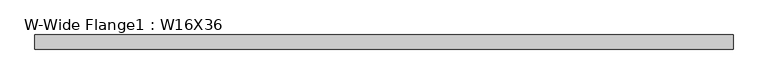
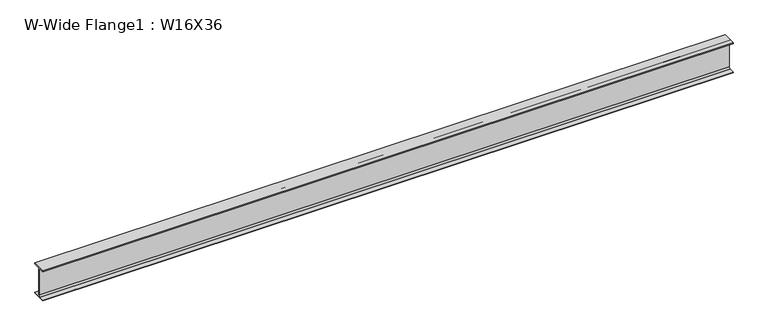
"""IFC4 building model written with IfcOpenShell, lengths in millimetres: beam geometry, W-Wide Flange1 : W16X36."""

from ifc_helpers import new_model, si_unit, point, frame, frame_2d, origin, place, context, project, spatial, polyline, circle_curve, trimmed, segment, composite_curve, outline, extrude, source, transform, mapped, element, save


def w_wide_flange1_w16x36_dd20d998(model_context):
    return source(origin(), model_context, "Body", "SweptSolid", [
        extrude(outline(composite_curve([segment(polyline([(88.773, -191.008), (88.773, -201.93), (-88.773, -201.93), (-88.773, -191.008), (-21.3995, -191.008)]), True, "CONTINUOUS"), segment(trimmed(circle_curve(frame_2d((-21.3995, -173.355)), 17.653), [point((-21.3995, -191.008))], [point((-3.7465, -173.355))], True, "CARTESIAN"), True, "CONTINUOUS"), segment(polyline([(-3.7465, -173.355), (-3.7465, 173.355)]), True, "CONTINUOUS"), segment(trimmed(circle_curve(frame_2d((-21.3995, 173.355)), 17.653), [point((-3.7465, 173.355))], [point((-21.3995, 191.008))], True, "CARTESIAN"), True, "CONTINUOUS"), segment(polyline([(-21.3995, 191.008), (-88.773, 191.008), (-88.773, 201.93), (88.773, 201.93), (88.773, 191.008), (21.3995, 191.008)]), True, "CONTINUOUS"), segment(trimmed(circle_curve(frame_2d((21.3995, 173.355)), 17.653), [point((21.3995, 191.008))], [point((3.7465, 173.355))], True, "CARTESIAN"), True, "CONTINUOUS"), segment(polyline([(3.7465, 173.355), (3.7465, -173.355)]), True, "CONTINUOUS"), segment(trimmed(circle_curve(frame_2d((21.3995, -173.355)), 17.653), [point((3.7465, -173.355))], [point((21.3995, -191.008))], True, "CARTESIAN"), True, "CONTINUOUS"), segment(polyline([(21.3995, -191.008), (88.773, -191.008)]), True, "CONTINUOUS")], self_intersect=False)), frame((-4399.7267802, 0.0, 0.0), z_axis=(1.0, 0.0, 0.0), x_axis=(0.0, 1.0, 0.0)), (0.0, 0.0, 1.0), 8787.9151819),
    ])


if __name__ == "__main__":
    model = new_model("IFC4")
    model_context = context("Model", 3, world=origin())
    ifc_project = project(units=[si_unit("LENGTHUNIT", "METRE", prefix="MILLI")], contexts=[model_context])
    site = spatial("IfcSite", under=ifc_project)
    building = spatial("IfcBuilding", under=site)
    placement = place(None, origin())
    w_wide_flange1_w16x36_shape = w_wide_flange1_w16x36_dd20d998(model_context)
    element("IfcBeam", 1, ObjectType="W-Wide Flange1 : W16X36", at=placement, inside=building, context=model_context, shape_type="MappedRepresentation", body=[
        mapped(w_wide_flange1_w16x36_shape, transform((0.0, 0.0, 0.0), x_axis=(1.0, 0.0, 0.0), y_axis=(0.0, 1.0, 0.0), z_axis=(0.0, 0.0, 1.0))),
    ])
    save(model, "model.ifc")

# Revit data of these elements
# Type "W-Wide Flange1 : W16X36"
#   Assembly Code = "B10"
#   W = 36
#   Start Extension Calculation [instance default] = 10' - 0"
#   Start Extension [instance default] = -0' - 0 1/2"
#   End Extension Calculation [instance default] = 10' - 0"
#   End Extension [instance default] = -0' - 0 1/2"
#   Length [instance default] = 5' - 0"
#   bf = 0' - 6.99"
#   d = 1' - 3.9"
#   k = 0' - 1 1/8"
#   k2 = 0' - 0.695"
#   tf = 0' - 0.43"
#   tw = 0' - 0.295"
#   A = 0.0736111 SF
#   Structural Material [instance default] = Metal - Steel - ASTM A992
# Element 1 (IfcBeam, "W-Wide Flange1 : W16X36")
#   Materials on its faces: "Metal - Steel - ASTM A992"
# Materials
#   "Metal - Steel - ASTM A992": class "Metal", colour RGB 199 199 199, transparency 0
